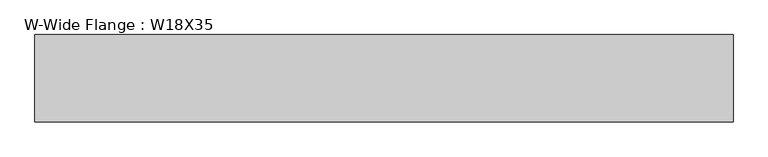
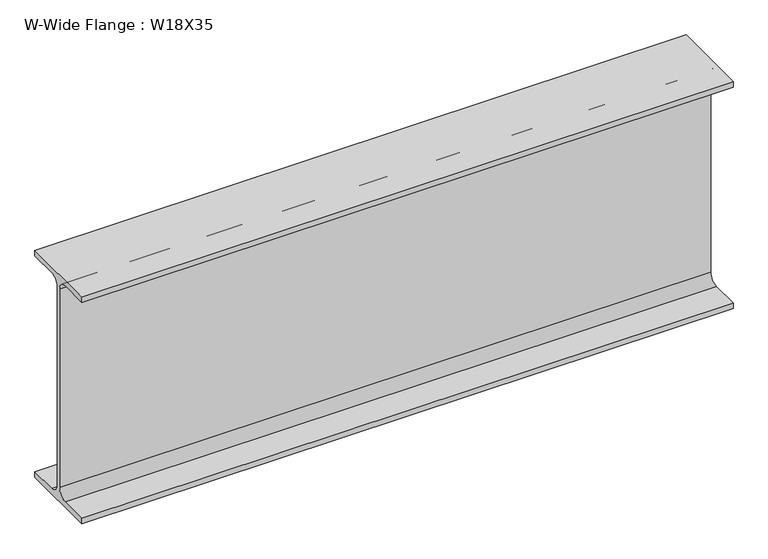
"""IFC4 building model written with IfcOpenShell, lengths in millimetres: beam geometry, W-Wide Flange : W18X35."""

from ifc_helpers import new_model, si_unit, point, frame, frame_2d, origin, place, context, project, spatial, polyline, circle_curve, trimmed, segment, composite_curve, outline, extrude, source, transform, mapped, element, save


def w_wide_flange_w18x35_2f775743(model_context):
    return source(origin(), model_context, "Body", "SweptSolid", [
        extrude(outline(composite_curve([segment(polyline([(76.2, -213.995), (76.2, -224.79), (-76.2, -224.79), (-76.2, -213.995), (-21.59, -213.995)]), True, "CONTINUOUS"), segment(trimmed(circle_curve(frame_2d((-21.59, -196.215)), 17.78), [point((-21.59, -213.995))], [point((-3.81, -196.215))], True, "CARTESIAN"), True, "CONTINUOUS"), segment(polyline([(-3.81, -196.215), (-3.81, 196.215)]), True, "CONTINUOUS"), segment(trimmed(circle_curve(frame_2d((-21.59, 196.215)), 17.78), [point((-3.81, 196.215))], [point((-21.59, 213.995))], True, "CARTESIAN"), True, "CONTINUOUS"), segment(polyline([(-21.59, 213.995), (-76.2, 213.995), (-76.2, 224.79), (76.2, 224.79), (76.2, 213.995), (21.59, 213.995)]), True, "CONTINUOUS"), segment(trimmed(circle_curve(frame_2d((21.59, 196.215)), 17.78), [point((21.59, 213.995))], [point((3.81, 196.215))], True, "CARTESIAN"), True, "CONTINUOUS"), segment(polyline([(3.81, 196.215), (3.81, -196.215)]), True, "CONTINUOUS"), segment(trimmed(circle_curve(frame_2d((21.59, -196.215)), 17.78), [point((3.81, -196.215))], [point((21.59, -213.995))], True, "CARTESIAN"), True, "CONTINUOUS"), segment(polyline([(21.59, -213.995), (76.2, -213.995)]), True, "CONTINUOUS")], self_intersect=False)), frame((-609.6, 0.0, 0.0), z_axis=(1.0, 0.0, 0.0), x_axis=(0.0, 1.0, 0.0)), (0.0, 0.0, 1.0), 1219.2),
    ])


if __name__ == "__main__":
    model = new_model("IFC4")
    model_context = context("Model", 3, world=origin())
    ifc_project = project(units=[si_unit("LENGTHUNIT", "METRE", prefix="MILLI")], contexts=[model_context])
    site = spatial("IfcSite", under=ifc_project)
    building = spatial("IfcBuilding", under=site)
    placement = place(None, origin())
    w_wide_flange_w18x35_shape = w_wide_flange_w18x35_2f775743(model_context)
    element("IfcBeam", 1, ObjectType="W-Wide Flange : W18X35", at=placement, inside=building, context=model_context, shape_type="MappedRepresentation", body=[
        mapped(w_wide_flange_w18x35_shape, transform((0.0, 0.0, 0.0), x_axis=(1.0, 0.0, 0.0), y_axis=(0.0, 1.0, 0.0), z_axis=(0.0, 0.0, 1.0))),
    ])
    save(model, "model.ifc")

# Revit data of these elements
# Type "W-Wide Flange : W18X35"
#   Assembly Code = "B10"
#   W = 35
#   Length [instance default] = 5' - 0"
#   bf = 0' - 6"
#   d = 1' - 5.7"
#   k = 0' - 1 1/8"
#   k2 = 0' - 0.7"
#   tf = 0' - 0.425"
#   tw = 0' - 0.3"
#   A = 0.0715278 SF
#   Structural Material [instance default] = Steel ASTM A992
# Element 1 (IfcBeam, "W-Wide Flange : W18X35")
#   Materials on its faces: "Steel ASTM A992"
# Materials
#   "Steel ASTM A992": class "Metal", colour RGB 199 199 199, transparency 0, Description = "Structural steel 50ksi", Cost = 0
